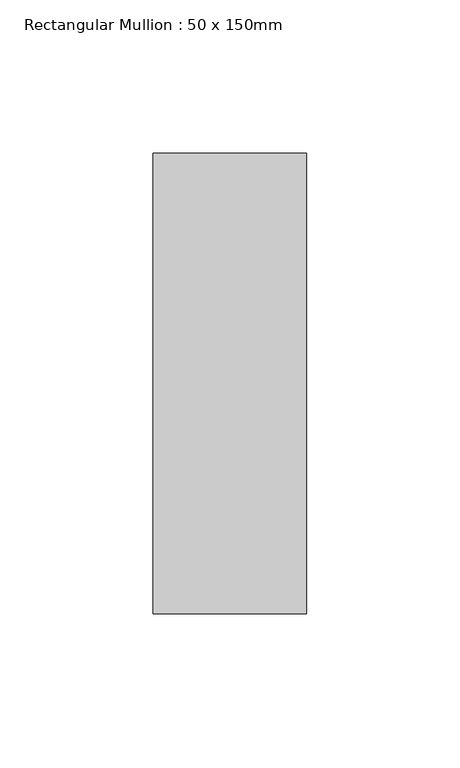
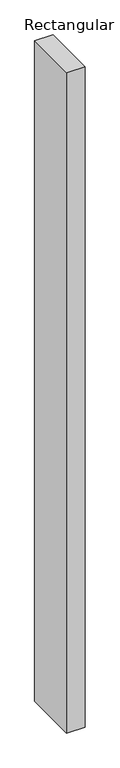
"""IFC4 building model written with IfcOpenShell, lengths in millimetres: member geometry, Rectangular Mullion : 50 x 150mm."""

from ifc_helpers import new_model, si_unit, frame, origin, place, context, project, spatial, polyline, outline, extrude, source, transform, mapped, element, save


def rectangular_mullion_50_x_150mm_5f4b7725(model_context):
    return source(origin(), model_context, "Body", "SweptSolid", [
        extrude(outline(polyline([(25.0, 75.0), (25.0, -75.0), (-25.0, -75.0), (-25.0, 75.0), (25.0, 75.0)])), frame((0.0, 0.0, -1899.9999997), z_axis=(0.0, 0.0, 1.0), x_axis=(1.0, 0.0, 0.0)), (0.0, 0.0, 1.0), 1899.9999997),
    ])


if __name__ == "__main__":
    model = new_model("IFC4")
    model_context = context("Model", 3, world=origin())
    ifc_project = project(units=[si_unit("LENGTHUNIT", "METRE", prefix="MILLI")], contexts=[model_context])
    site = spatial("IfcSite", under=ifc_project)
    building = spatial("IfcBuilding", under=site)
    placement = place(None, origin())
    rectangular_mullion_50_x_150mm_shape = rectangular_mullion_50_x_150mm_5f4b7725(model_context)
    element("IfcMember", 1, ObjectType="Rectangular Mullion : 50 x 150mm", at=placement, inside=building, context=model_context, shape_type="MappedRepresentation", body=[
        mapped(rectangular_mullion_50_x_150mm_shape, transform((0.0, 0.0, 0.0), x_axis=(1.0, 0.0, 0.0), y_axis=(0.0, 1.0, 0.0), z_axis=(0.0, 0.0, 1.0))),
    ])
    save(model, "model.ifc")

# Revit data of these elements
# Type "Rectangular Mullion : 50 x 150mm"
#   built-in parameter 1007304 = 0.492126 (stored number, unit not read)
#   built-in parameter 1007301 = 0.082021 (stored number, unit not read)
#   built-in parameter 1007300 = 0.082021 (stored number, unit not read)
# Element 1 (IfcMember, "Rectangular Mullion : 50 x 150mm")
#   Materials on its faces: "Metal - Aluminium"
# Materials
#   "Metal - Aluminium": class "Metal", colour RGB 247 247 247, transparency 0
